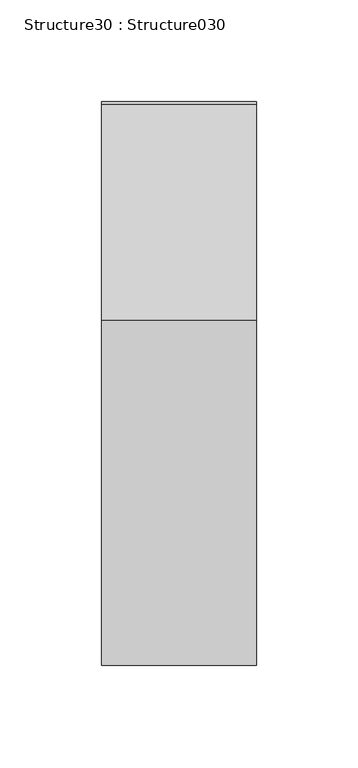
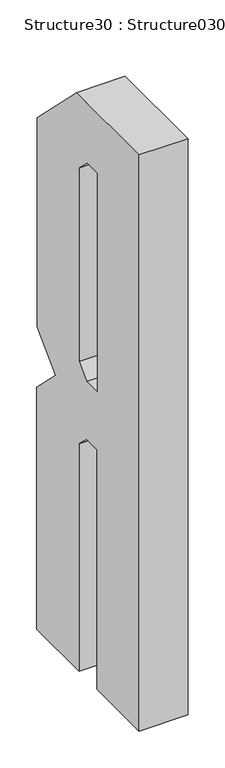
"""IFC4 building model written with IfcOpenShell, lengths in millimetres: proxy geometry, Structure30 : Structure030."""

import ifcopenshell
import ifcopenshell.guid

model = None  # the IFC model being written
_history = None  # IfcOwnerHistory: only IFC2X3 demands one
_inside = {}  # id of a spatial element -> (the spatial element, [elements in it])
_under = {}  # id of a project, library or spatial element -> (it, [spatial elements below it])
_declared = {}  # id of a project -> (the project, [libraries it declares])
_typed = {}  # id of a type object -> (the type object, [elements of that type])
_made_of = {}  # id of a material, layer set ... -> (it, [elements and type objects made of it])


def new_model(schema):
    """Start an empty IFC model of exactly this schema.

    Asked for "IFC4X3", IfcOpenShell would pick the latest addendum, in which some entities
    have other attributes; the version numbers below select the first issue.
    IFC2X3 requires an IfcOwnerHistory on every rooted entity: one is made here for all.
    """
    global model, _history
    if schema == "IFC4X3":
        model = ifcopenshell.file(schema_version=(4, 3, 0, 0))
    else:
        model = ifcopenshell.file(schema=schema)
    _inside.clear()
    _under.clear()
    _declared.clear()
    _typed.clear()
    _made_of.clear()
    _history = None
    if model.schema == "IFC2X3":
        org = make("IfcOrganization", Name="unknown")
        user = make(
            "IfcPersonAndOrganization",
            ThePerson=make("IfcPerson", FamilyName="unknown"),
            TheOrganization=org,
        )
        app = make(
            "IfcApplication",
            ApplicationDeveloper=org,
            Version="unknown",
            ApplicationFullName="unknown",
            ApplicationIdentifier="unknown",
        )
        _history = make(
            "IfcOwnerHistory",
            OwningUser=user,
            OwningApplication=app,
            ChangeAction="ADDED",
            CreationDate=0,
        )
    return model


def make(cls, **values):
    """One entity of the class cls with the attributes given. An attribute that is None is left unset."""
    return model.create_entity(
        cls, **{name: value for name, value in values.items() if value is not None}
    )


def rooted(cls, **values):
    """An entity with a GlobalId (a new one), such as an element, a storey or a relation."""
    return make(cls, GlobalId=ifcopenshell.guid.new(), OwnerHistory=_history, **values)


def si_unit(unit_type, name, prefix=None):
    """IfcSIUnit, for example si_unit("LENGTHUNIT", "METRE", prefix="MILLI")."""
    return make("IfcSIUnit", UnitType=unit_type, Prefix=prefix, Name=name)


def assignment(units):
    """IfcUnitAssignment: the units of a project."""
    return None if units is None else make("IfcUnitAssignment", Units=units)


def point(xyz):
    """IfcCartesianPoint."""
    return None if xyz is None else make("IfcCartesianPoint", Coordinates=xyz)


def direction(xyz):
    """IfcDirection."""
    return None if xyz is None else make("IfcDirection", DirectionRatios=xyz)


def frame(location, z_axis=None, x_axis=None):
    """IfcAxis2Placement3D, a coordinate frame: its origin and axes. An axis left out is left unset."""
    return make(
        "IfcAxis2Placement3D",
        Location=point(location),
        Axis=direction(z_axis),
        RefDirection=direction(x_axis),
    )


def origin():
    """The frame at (0, 0, 0) with its axes left unset."""
    return frame((0.0, 0.0, 0.0))


def place(relative_to, where):
    """IfcLocalPlacement: puts the frame where relative to a parent placement (None: the world)."""
    return make(
        "IfcLocalPlacement", PlacementRelTo=relative_to, RelativePlacement=where
    )


def context(
    kind, dimensions, precision=None, world=None, true_north=None, identifier=None
):
    """IfcGeometricRepresentationContext, for example the 3D "Model" context."""
    return make(
        "IfcGeometricRepresentationContext",
        ContextIdentifier=identifier,
        ContextType=kind,
        CoordinateSpaceDimension=dimensions,
        Precision=precision,
        WorldCoordinateSystem=world,
        TrueNorth=true_north,
    )


def project(units=None, contexts=None):
    """IfcProject with its units and contexts."""
    return rooted(
        "IfcProject",
        Name="project",
        RepresentationContexts=contexts,
        UnitsInContext=assignment(units),
    )


def spatial(cls, under=None, at=None, **own):
    """A site, building, storey or space (cls), placed at a placement, below another one or the project."""
    s = rooted(cls, ObjectPlacement=at, **own)
    if under is not None:
        _under.setdefault(under.id(), (under, []))[1].append(s)
    return s


def polyline(points):
    """IfcPolyline through the points."""
    return make("IfcPolyline", Points=[point(p) for p in points])


def outline(outer, holes=None, kind="AREA"):
    """IfcArbitraryClosedProfileDef: a profile drawn as a closed curve; with holes, ...WithVoids."""
    if holes is None:
        return make("IfcArbitraryClosedProfileDef", ProfileType=kind, OuterCurve=outer)
    return make(
        "IfcArbitraryProfileDefWithVoids",
        ProfileType=kind,
        OuterCurve=outer,
        InnerCurves=holes,
    )


def extrude(swept, where, along, depth):
    """IfcExtrudedAreaSolid: the profile swept, set in the frame where, extruded along a direction by depth."""
    return make(
        "IfcExtrudedAreaSolid",
        SweptArea=swept,
        Position=where,
        ExtrudedDirection=direction(along),
        Depth=depth,
    )


def shape(context_of_items, identifier, shape_type, items):
    """IfcShapeRepresentation: the items that make up one representation, for example the "Body"."""
    return make(
        "IfcShapeRepresentation",
        ContextOfItems=context_of_items,
        RepresentationIdentifier=identifier,
        RepresentationType=shape_type,
        Items=items,
    )


def source(mapping_origin, context_of_items, identifier, shape_type, items):
    """IfcRepresentationMap: a shape defined once, which mapped items show again and again."""
    return make(
        "IfcRepresentationMap",
        MappingOrigin=mapping_origin,
        MappedRepresentation=shape(context_of_items, identifier, shape_type, items),
    )


def transform(
    local_origin,
    x_axis=None,
    y_axis=None,
    z_axis=None,
    scale=None,
    scale2=None,
    scale3=None,
    uniform=True,
):
    """IfcCartesianTransformationOperator3D, or its non-uniform kind. x_axis, y_axis, z_axis: its Axis1, 2, 3."""
    if uniform:
        return make(
            "IfcCartesianTransformationOperator3D",
            Axis1=direction(x_axis),
            Axis2=direction(y_axis),
            LocalOrigin=point(local_origin),
            Scale=scale,
            Axis3=direction(z_axis),
        )
    return make(
        "IfcCartesianTransformationOperator3DnonUniform",
        Axis1=direction(x_axis),
        Axis2=direction(y_axis),
        LocalOrigin=point(local_origin),
        Scale=scale,
        Axis3=direction(z_axis),
        Scale2=scale2,
        Scale3=scale3,
    )


def mapped(mapping_source, mapping_target):
    """IfcMappedItem: shows the shape of a source again, moved by a transform."""
    return make(
        "IfcMappedItem", MappingSource=mapping_source, MappingTarget=mapping_target
    )


def made_of(thing, what):
    """Note that an element or type object is made of a material, layer set ...; save() writes the relation."""
    if what is not None:
        _made_of.setdefault(what.id(), (what, []))[1].append(thing)
    return thing


def element(
    cls,
    number,
    at=None,
    inside=None,
    cuts=None,
    type_object=None,
    material=None,
    context=None,
    identifier="Body",
    shape_type=None,
    held_by="IfcProductDefinitionShape",
    body=None,
    shapes=None,
    **own,
):
    """One element of the class cls, such as IfcWall. Its Tag is "e" and its number.

    at: its placement. inside: the storey or other place that contains it. cuts: it is an
    opening in that element (IfcRelVoidsElement). A single representation is given by context,
    identifier, shape_type and body (its items); several are given by shapes. held_by: the class
    of the entity that holds the representations. save() writes the other relations.
    """
    e = rooted(cls, Tag="e%d" % number, ObjectPlacement=at, **own)
    if body is not None:
        shapes = [shape(context, identifier, shape_type, body)]
    if shapes is not None:
        e.Representation = make(held_by, Representations=shapes)
    if inside is not None:
        _inside.setdefault(inside.id(), (inside, []))[1].append(e)
    if cuts is not None:
        rooted(
            "IfcRelVoidsElement", RelatingBuildingElement=cuts, RelatedOpeningElement=e
        )
    if type_object is not None:
        _typed.setdefault(type_object.id(), (type_object, []))[1].append(e)
    return made_of(e, material)


def aggregate(whole, parts):
    """IfcRelAggregates: a whole, such as a stair, and the parts it consists of."""
    return rooted("IfcRelAggregates", RelatingObject=whole, RelatedObjects=parts)


def save(model, path):
    """Write the relations noted so far, then the file.

    IfcRelAggregates (storeys below a building ...), IfcRelContainedInSpatialStructure (elements
    in a storey), IfcRelDefinesByType, IfcRelAssociatesMaterial and IfcRelDeclares: one each for
    every whole, place, type object, material and project.
    """
    for whole, parts in _under.values():
        aggregate(whole, parts)
    for where, things in _inside.values():
        rooted(
            "IfcRelContainedInSpatialStructure",
            RelatedElements=things,
            RelatingStructure=where,
        )
    for kind, things in _typed.values():
        rooted("IfcRelDefinesByType", RelatedObjects=things, RelatingType=kind)
    for what, things in _made_of.values():
        rooted("IfcRelAssociatesMaterial", RelatedObjects=things, RelatingMaterial=what)
    for by, libraries in _declared.values():
        rooted("IfcRelDeclares", RelatingContext=by, RelatedDefinitions=libraries)
    model.write(path)


def structure30_structure030_552ecfaa(model_context):
    return source(origin(), model_context, "Body", "SweptSolid", [
        extrude(outline(polyline([(251331.4415394, 4374.3842509), (251331.4415394, 4028.9992538), (251282.4933618, 3978.6781441), (251332.8144715, 3928.3570344), (251332.8144715, 3528.5825142), (251218.5789649, 3528.5825142), (251218.5789649, 3903.8911328), (251198.1808469, 3924.2892507), (251169.6213405, 3924.2892507), (251169.6213405, 3528.5825142), (251055.411655, 3528.5825142), (251055.411655, 4480.4419946), (251225.3837957, 4480.4419946), (251331.4415394, 4374.3842509)]), holes=[polyline([(251169.6213405, 4020.827159), (251196.8223999, 4020.827159), (251217.223037, 4041.2277961), (251217.223037, 4360.7915935), (251196.824919, 4381.1897115), (251169.6213405, 4381.1897115), (251169.6213405, 4020.827159)])]), frame((-38594.2176606, 0.0, 0.0), z_axis=(1.0, 0.0, 0.0), x_axis=(0.0, 1.0, 0.0)), (0.0, 0.0, 1.0), 76.2),
    ])


if __name__ == "__main__":
    model = new_model("IFC4")
    model_context = context("Model", 3, world=origin())
    ifc_project = project(units=[si_unit("LENGTHUNIT", "METRE", prefix="MILLI")], contexts=[model_context])
    site = spatial("IfcSite", under=ifc_project)
    building = spatial("IfcBuilding", under=site)
    placement = place(None, origin())
    structure30_structure030_shape = structure30_structure030_552ecfaa(model_context)
    element("IfcBuildingElementProxy", 1, Name="Structure30 : Structure030", ObjectType="Structure30 : Structure030", at=placement, inside=building, context=model_context, shape_type="MappedRepresentation", body=[
        mapped(structure30_structure030_shape, transform((0.0, 0.0, 0.0), x_axis=(1.0, 0.0, 0.0), y_axis=(0.0, 1.0, 0.0), z_axis=(0.0, 0.0, 1.0))),
    ])
    save(model, "model.ifc")

# Revit data of these elements
# Type "Structure30 : Structure030"
#   NameOverride = "Structure030"
# Element 1 (IfcBuildingElementProxy, "Structure30 : Structure030")
#   Materials on its faces: "BRUSHED ALUM. LETTERING"
# Materials
#   "BRUSHED ALUM. LETTERING": class "Unassigned", colour RGB 169 181 186, transparency 0, Cost = 0
